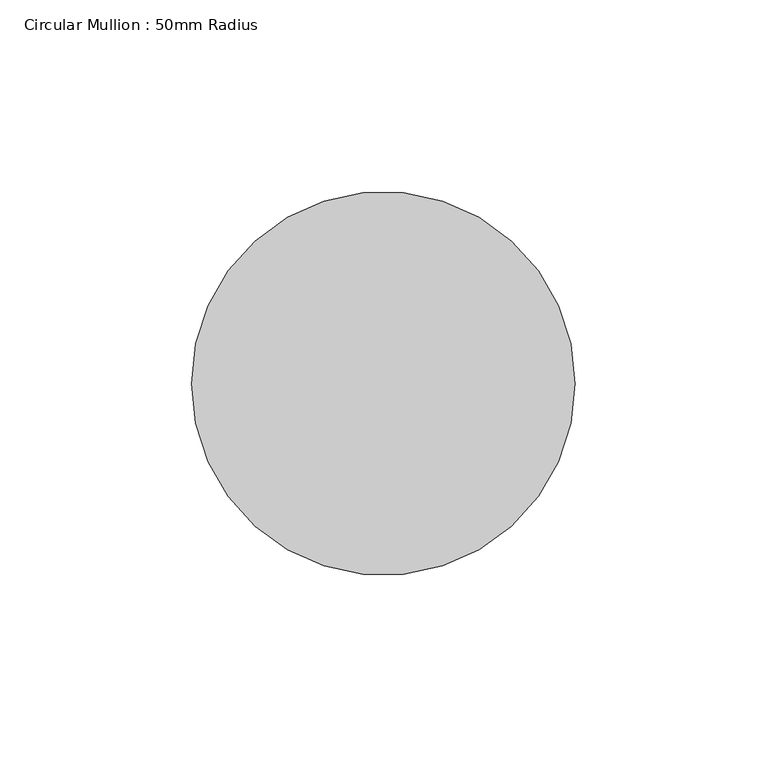
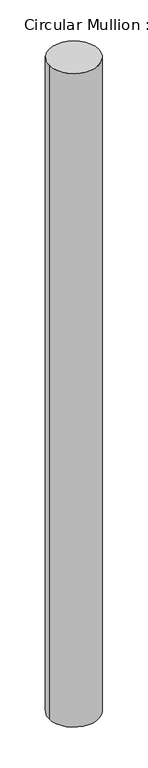
"""IFC4 building model written with IfcOpenShell, lengths in millimetres: member geometry, Circular Mullion : 50mm Radius."""

from ifc_helpers import new_model, si_unit, point, frame, origin, origin_2d, place, context, project, spatial, circle_curve, trimmed, segment, composite_curve, outline, extrude, source, transform, mapped, element, save


def circular_mullion_50mm_radius_74eeb39e(model_context):
    return source(origin(), model_context, "Body", "SweptSolid", [
        extrude(outline(composite_curve([segment(trimmed(circle_curve(origin_2d(), 50.0), [point((50.0, 0.0))], [point((-50.0, 0.0))], False, "CARTESIAN"), True, "CONTINUOUS"), segment(trimmed(circle_curve(origin_2d(), 50.0), [point((-50.0, 0.0))], [point((50.0, 0.0))], False, "CARTESIAN"), True, "CONTINUOUS")], self_intersect=False)), frame((0.0, 0.0, -1399.0414938), z_axis=(0.0, 0.0, 1.0), x_axis=(1.0, 0.0, 0.0)), (0.0, 0.0, 1.0), 1399.0414938),
    ])


if __name__ == "__main__":
    model = new_model("IFC4")
    model_context = context("Model", 3, world=origin())
    ifc_project = project(units=[si_unit("LENGTHUNIT", "METRE", prefix="MILLI")], contexts=[model_context])
    site = spatial("IfcSite", under=ifc_project)
    building = spatial("IfcBuilding", under=site)
    placement = place(None, origin())
    circular_mullion_50mm_radius_shape = circular_mullion_50mm_radius_74eeb39e(model_context)
    element("IfcMember", 1, ObjectType="Circular Mullion : 50mm Radius", at=placement, inside=building, context=model_context, shape_type="MappedRepresentation", body=[
        mapped(circular_mullion_50mm_radius_shape, transform((0.0, 0.0, 0.0), x_axis=(1.0, 0.0, 0.0), y_axis=(0.0, 1.0, 0.0), z_axis=(0.0, 0.0, 1.0))),
    ])
    save(model, "model.ifc")

# Revit data of these elements
# Type "Circular Mullion : 50mm Radius"
#   built-in parameter 1007350 = 0.164042 (stored number, unit not read)
# Element 1 (IfcMember, "Circular Mullion : 50mm Radius")
#   Materials on its faces: "Aluminium"
# Materials
#   "Aluminium": class "Metal", colour RGB 247 247 247, transparency 0, Description = "Aluminium 6061", Cost = 0
